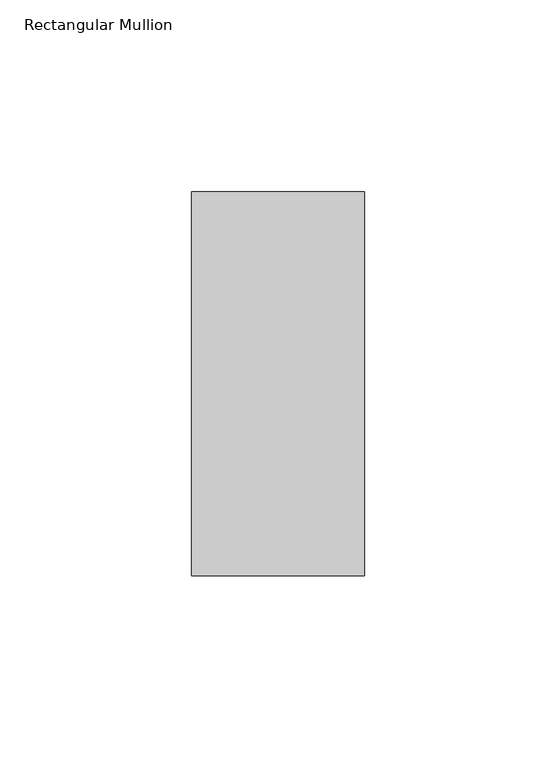
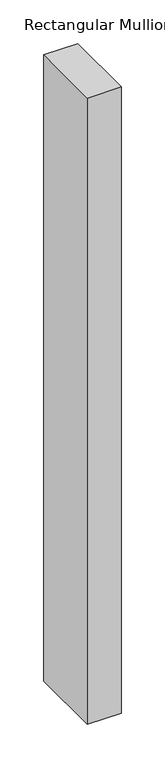
"""IFC4 building model written with IfcOpenShell, lengths in millimetres: member geometry, Rectangular Mullion : 알루미늄_Rectangular Cap_100 x 45."""

import ifcopenshell
import ifcopenshell.guid

model = None  # the IFC model being written
_history = None  # IfcOwnerHistory: only IFC2X3 demands one
_inside = {}  # id of a spatial element -> (the spatial element, [elements in it])
_under = {}  # id of a project, library or spatial element -> (it, [spatial elements below it])
_declared = {}  # id of a project -> (the project, [libraries it declares])
_typed = {}  # id of a type object -> (the type object, [elements of that type])
_made_of = {}  # id of a material, layer set ... -> (it, [elements and type objects made of it])


def new_model(schema):
    """Start an empty IFC model of exactly this schema.

    Asked for "IFC4X3", IfcOpenShell would pick the latest addendum, in which some entities
    have other attributes; the version numbers below select the first issue.
    IFC2X3 requires an IfcOwnerHistory on every rooted entity: one is made here for all.
    """
    global model, _history
    if schema == "IFC4X3":
        model = ifcopenshell.file(schema_version=(4, 3, 0, 0))
    else:
        model = ifcopenshell.file(schema=schema)
    _inside.clear()
    _under.clear()
    _declared.clear()
    _typed.clear()
    _made_of.clear()
    _history = None
    if model.schema == "IFC2X3":
        org = make("IfcOrganization", Name="unknown")
        user = make(
            "IfcPersonAndOrganization",
            ThePerson=make("IfcPerson", FamilyName="unknown"),
            TheOrganization=org,
        )
        app = make(
            "IfcApplication",
            ApplicationDeveloper=org,
            Version="unknown",
            ApplicationFullName="unknown",
            ApplicationIdentifier="unknown",
        )
        _history = make(
            "IfcOwnerHistory",
            OwningUser=user,
            OwningApplication=app,
            ChangeAction="ADDED",
            CreationDate=0,
        )
    return model


def make(cls, **values):
    """One entity of the class cls with the attributes given. An attribute that is None is left unset."""
    return model.create_entity(
        cls, **{name: value for name, value in values.items() if value is not None}
    )


def rooted(cls, **values):
    """An entity with a GlobalId (a new one), such as an element, a storey or a relation."""
    return make(cls, GlobalId=ifcopenshell.guid.new(), OwnerHistory=_history, **values)


def si_unit(unit_type, name, prefix=None):
    """IfcSIUnit, for example si_unit("LENGTHUNIT", "METRE", prefix="MILLI")."""
    return make("IfcSIUnit", UnitType=unit_type, Prefix=prefix, Name=name)


def assignment(units):
    """IfcUnitAssignment: the units of a project."""
    return None if units is None else make("IfcUnitAssignment", Units=units)


def point(xyz):
    """IfcCartesianPoint."""
    return None if xyz is None else make("IfcCartesianPoint", Coordinates=xyz)


def direction(xyz):
    """IfcDirection."""
    return None if xyz is None else make("IfcDirection", DirectionRatios=xyz)


def frame(location, z_axis=None, x_axis=None):
    """IfcAxis2Placement3D, a coordinate frame: its origin and axes. An axis left out is left unset."""
    return make(
        "IfcAxis2Placement3D",
        Location=point(location),
        Axis=direction(z_axis),
        RefDirection=direction(x_axis),
    )


def origin():
    """The frame at (0, 0, 0) with its axes left unset."""
    return frame((0.0, 0.0, 0.0))


def place(relative_to, where):
    """IfcLocalPlacement: puts the frame where relative to a parent placement (None: the world)."""
    return make(
        "IfcLocalPlacement", PlacementRelTo=relative_to, RelativePlacement=where
    )


def context(
    kind, dimensions, precision=None, world=None, true_north=None, identifier=None
):
    """IfcGeometricRepresentationContext, for example the 3D "Model" context."""
    return make(
        "IfcGeometricRepresentationContext",
        ContextIdentifier=identifier,
        ContextType=kind,
        CoordinateSpaceDimension=dimensions,
        Precision=precision,
        WorldCoordinateSystem=world,
        TrueNorth=true_north,
    )


def project(units=None, contexts=None):
    """IfcProject with its units and contexts."""
    return rooted(
        "IfcProject",
        Name="project",
        RepresentationContexts=contexts,
        UnitsInContext=assignment(units),
    )


def spatial(cls, under=None, at=None, **own):
    """A site, building, storey or space (cls), placed at a placement, below another one or the project."""
    s = rooted(cls, ObjectPlacement=at, **own)
    if under is not None:
        _under.setdefault(under.id(), (under, []))[1].append(s)
    return s


def polyline(points):
    """IfcPolyline through the points."""
    return make("IfcPolyline", Points=[point(p) for p in points])


def outline(outer, holes=None, kind="AREA"):
    """IfcArbitraryClosedProfileDef: a profile drawn as a closed curve; with holes, ...WithVoids."""
    if holes is None:
        return make("IfcArbitraryClosedProfileDef", ProfileType=kind, OuterCurve=outer)
    return make(
        "IfcArbitraryProfileDefWithVoids",
        ProfileType=kind,
        OuterCurve=outer,
        InnerCurves=holes,
    )


def extrude(swept, where, along, depth):
    """IfcExtrudedAreaSolid: the profile swept, set in the frame where, extruded along a direction by depth."""
    return make(
        "IfcExtrudedAreaSolid",
        SweptArea=swept,
        Position=where,
        ExtrudedDirection=direction(along),
        Depth=depth,
    )


def shape(context_of_items, identifier, shape_type, items):
    """IfcShapeRepresentation: the items that make up one representation, for example the "Body"."""
    return make(
        "IfcShapeRepresentation",
        ContextOfItems=context_of_items,
        RepresentationIdentifier=identifier,
        RepresentationType=shape_type,
        Items=items,
    )


def source(mapping_origin, context_of_items, identifier, shape_type, items):
    """IfcRepresentationMap: a shape defined once, which mapped items show again and again."""
    return make(
        "IfcRepresentationMap",
        MappingOrigin=mapping_origin,
        MappedRepresentation=shape(context_of_items, identifier, shape_type, items),
    )


def transform(
    local_origin,
    x_axis=None,
    y_axis=None,
    z_axis=None,
    scale=None,
    scale2=None,
    scale3=None,
    uniform=True,
):
    """IfcCartesianTransformationOperator3D, or its non-uniform kind. x_axis, y_axis, z_axis: its Axis1, 2, 3."""
    if uniform:
        return make(
            "IfcCartesianTransformationOperator3D",
            Axis1=direction(x_axis),
            Axis2=direction(y_axis),
            LocalOrigin=point(local_origin),
            Scale=scale,
            Axis3=direction(z_axis),
        )
    return make(
        "IfcCartesianTransformationOperator3DnonUniform",
        Axis1=direction(x_axis),
        Axis2=direction(y_axis),
        LocalOrigin=point(local_origin),
        Scale=scale,
        Axis3=direction(z_axis),
        Scale2=scale2,
        Scale3=scale3,
    )


def mapped(mapping_source, mapping_target):
    """IfcMappedItem: shows the shape of a source again, moved by a transform."""
    return make(
        "IfcMappedItem", MappingSource=mapping_source, MappingTarget=mapping_target
    )


def made_of(thing, what):
    """Note that an element or type object is made of a material, layer set ...; save() writes the relation."""
    if what is not None:
        _made_of.setdefault(what.id(), (what, []))[1].append(thing)
    return thing


def element(
    cls,
    number,
    at=None,
    inside=None,
    cuts=None,
    type_object=None,
    material=None,
    context=None,
    identifier="Body",
    shape_type=None,
    held_by="IfcProductDefinitionShape",
    body=None,
    shapes=None,
    **own,
):
    """One element of the class cls, such as IfcWall. Its Tag is "e" and its number.

    at: its placement. inside: the storey or other place that contains it. cuts: it is an
    opening in that element (IfcRelVoidsElement). A single representation is given by context,
    identifier, shape_type and body (its items); several are given by shapes. held_by: the class
    of the entity that holds the representations. save() writes the other relations.
    """
    e = rooted(cls, Tag="e%d" % number, ObjectPlacement=at, **own)
    if body is not None:
        shapes = [shape(context, identifier, shape_type, body)]
    if shapes is not None:
        e.Representation = make(held_by, Representations=shapes)
    if inside is not None:
        _inside.setdefault(inside.id(), (inside, []))[1].append(e)
    if cuts is not None:
        rooted(
            "IfcRelVoidsElement", RelatingBuildingElement=cuts, RelatedOpeningElement=e
        )
    if type_object is not None:
        _typed.setdefault(type_object.id(), (type_object, []))[1].append(e)
    return made_of(e, material)


def aggregate(whole, parts):
    """IfcRelAggregates: a whole, such as a stair, and the parts it consists of."""
    return rooted("IfcRelAggregates", RelatingObject=whole, RelatedObjects=parts)


def save(model, path):
    """Write the relations noted so far, then the file.

    IfcRelAggregates (storeys below a building ...), IfcRelContainedInSpatialStructure (elements
    in a storey), IfcRelDefinesByType, IfcRelAssociatesMaterial and IfcRelDeclares: one each for
    every whole, place, type object, material and project.
    """
    for whole, parts in _under.values():
        aggregate(whole, parts)
    for where, things in _inside.values():
        rooted(
            "IfcRelContainedInSpatialStructure",
            RelatedElements=things,
            RelatingStructure=where,
        )
    for kind, things in _typed.values():
        rooted("IfcRelDefinesByType", RelatedObjects=things, RelatingType=kind)
    for what, things in _made_of.values():
        rooted("IfcRelAssociatesMaterial", RelatedObjects=things, RelatingMaterial=what)
    for by, libraries in _declared.values():
        rooted("IfcRelDeclares", RelatingContext=by, RelatedDefinitions=libraries)
    model.write(path)


def rectangular_mullion_c63874d8(model_context):
    return source(origin(), model_context, "Body", "SweptSolid", [
        extrude(outline(polyline([(0.0, 50.0), (0.0, -50.0), (-45.0, -50.0), (-45.0, 50.0), (0.0, 50.0)])), frame((0.0, 0.0, -877.5), z_axis=(0.0, 0.0, 1.0), x_axis=(1.0, 0.0, 0.0)), (0.0, 0.0, 1.0), 877.5),
    ])


if __name__ == "__main__":
    model = new_model("IFC4")
    model_context = context("Model", 3, world=origin())
    ifc_project = project(units=[si_unit("LENGTHUNIT", "METRE", prefix="MILLI")], contexts=[model_context])
    site = spatial("IfcSite", under=ifc_project)
    building = spatial("IfcBuilding", under=site)
    placement = place(None, origin())
    rectangular_mullion_shape = rectangular_mullion_c63874d8(model_context)
    element("IfcMember", 1, ObjectType="Rectangular Mullion : 알루미늄_Rectangular Cap_100 x 45", at=placement, inside=building, context=model_context, shape_type="MappedRepresentation", body=[
        mapped(rectangular_mullion_shape, transform((0.0, 0.0, 0.0), x_axis=(1.0, 0.0, 0.0), y_axis=(0.0, 1.0, 0.0), z_axis=(0.0, 0.0, 1.0))),
    ])
    save(model, "model.ifc")

# Revit data of these elements
# Type "Rectangular Mullion : 알루미늄_Rectangular Cap_100 x 45"
#   built-in parameter 1007304 = 0.328084 (stored number, unit not read)
#   built-in parameter 1007301 = 0.0738189 (stored number, unit not read)
#   built-in parameter 1007300 = 0.0738189 (stored number, unit not read)
# Element 1 (IfcMember, "Rectangular Mullion : 알루미늄_Rectangular Cap_100 x 45")
#   Materials on its faces: "00_Metal_Stainless Steel"
# Materials
#   "00_Metal_Stainless Steel": class "Metal", colour RGB 148 148 148, transparency 0, Description = "Steel", Cost = 0
